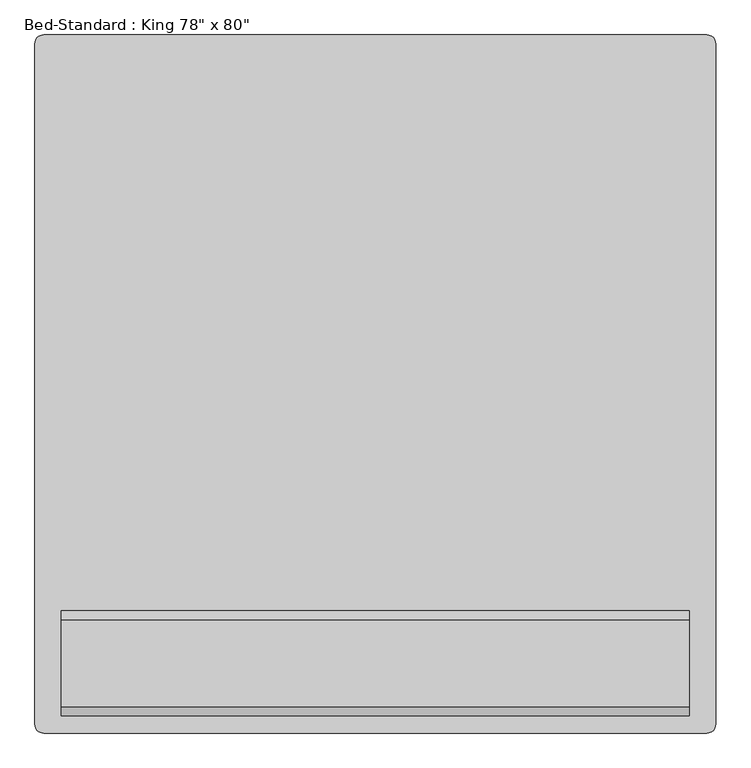
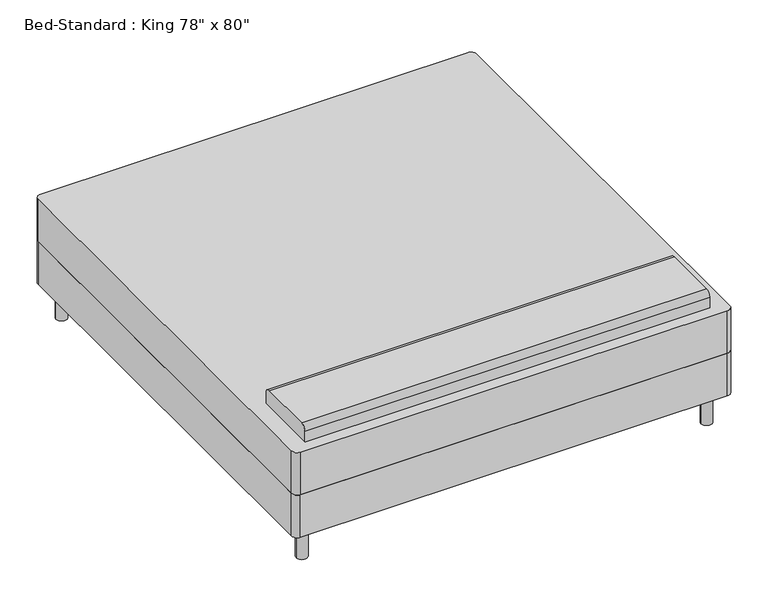
"""IFC4 building model written with IfcOpenShell, lengths in millimetres: furniture geometry."""

import ifcopenshell
import ifcopenshell.guid

model = None  # the IFC model being written
_history = None  # IfcOwnerHistory: only IFC2X3 demands one
_inside = {}  # id of a spatial element -> (the spatial element, [elements in it])
_under = {}  # id of a project, library or spatial element -> (it, [spatial elements below it])
_declared = {}  # id of a project -> (the project, [libraries it declares])
_typed = {}  # id of a type object -> (the type object, [elements of that type])
_made_of = {}  # id of a material, layer set ... -> (it, [elements and type objects made of it])


def new_model(schema):
    """Start an empty IFC model of exactly this schema.

    Asked for "IFC4X3", IfcOpenShell would pick the latest addendum, in which some entities
    have other attributes; the version numbers below select the first issue.
    IFC2X3 requires an IfcOwnerHistory on every rooted entity: one is made here for all.
    """
    global model, _history
    if schema == "IFC4X3":
        model = ifcopenshell.file(schema_version=(4, 3, 0, 0))
    else:
        model = ifcopenshell.file(schema=schema)
    _inside.clear()
    _under.clear()
    _declared.clear()
    _typed.clear()
    _made_of.clear()
    _history = None
    if model.schema == "IFC2X3":
        org = make("IfcOrganization", Name="unknown")
        user = make(
            "IfcPersonAndOrganization",
            ThePerson=make("IfcPerson", FamilyName="unknown"),
            TheOrganization=org,
        )
        app = make(
            "IfcApplication",
            ApplicationDeveloper=org,
            Version="unknown",
            ApplicationFullName="unknown",
            ApplicationIdentifier="unknown",
        )
        _history = make(
            "IfcOwnerHistory",
            OwningUser=user,
            OwningApplication=app,
            ChangeAction="ADDED",
            CreationDate=0,
        )
    return model


def make(cls, **values):
    """One entity of the class cls with the attributes given. An attribute that is None is left unset."""
    return model.create_entity(
        cls, **{name: value for name, value in values.items() if value is not None}
    )


def rooted(cls, **values):
    """An entity with a GlobalId (a new one), such as an element, a storey or a relation."""
    return make(cls, GlobalId=ifcopenshell.guid.new(), OwnerHistory=_history, **values)


def si_unit(unit_type, name, prefix=None):
    """IfcSIUnit, for example si_unit("LENGTHUNIT", "METRE", prefix="MILLI")."""
    return make("IfcSIUnit", UnitType=unit_type, Prefix=prefix, Name=name)


def assignment(units):
    """IfcUnitAssignment: the units of a project."""
    return None if units is None else make("IfcUnitAssignment", Units=units)


def point(xyz):
    """IfcCartesianPoint."""
    return None if xyz is None else make("IfcCartesianPoint", Coordinates=xyz)


def direction(xyz):
    """IfcDirection."""
    return None if xyz is None else make("IfcDirection", DirectionRatios=xyz)


def frame(location, z_axis=None, x_axis=None):
    """IfcAxis2Placement3D, a coordinate frame: its origin and axes. An axis left out is left unset."""
    return make(
        "IfcAxis2Placement3D",
        Location=point(location),
        Axis=direction(z_axis),
        RefDirection=direction(x_axis),
    )


def frame_2d(location, x_axis=None):
    """IfcAxis2Placement2D, a coordinate frame in the plane: its origin and x axis."""
    return make(
        "IfcAxis2Placement2D", Location=point(location), RefDirection=direction(x_axis)
    )


def origin():
    """The frame at (0, 0, 0) with its axes left unset."""
    return frame((0.0, 0.0, 0.0))


def origin_with_axes():
    """The frame at (0, 0, 0) with the z axis (0, 0, 1) and the x axis (1, 0, 0) written out."""
    return frame((0.0, 0.0, 0.0), z_axis=(0.0, 0.0, 1.0), x_axis=(1.0, 0.0, 0.0))


def place(relative_to, where):
    """IfcLocalPlacement: puts the frame where relative to a parent placement (None: the world)."""
    return make(
        "IfcLocalPlacement", PlacementRelTo=relative_to, RelativePlacement=where
    )


def context(
    kind, dimensions, precision=None, world=None, true_north=None, identifier=None
):
    """IfcGeometricRepresentationContext, for example the 3D "Model" context."""
    return make(
        "IfcGeometricRepresentationContext",
        ContextIdentifier=identifier,
        ContextType=kind,
        CoordinateSpaceDimension=dimensions,
        Precision=precision,
        WorldCoordinateSystem=world,
        TrueNorth=true_north,
    )


def project(units=None, contexts=None):
    """IfcProject with its units and contexts."""
    return rooted(
        "IfcProject",
        Name="project",
        RepresentationContexts=contexts,
        UnitsInContext=assignment(units),
    )


def spatial(cls, under=None, at=None, **own):
    """A site, building, storey or space (cls), placed at a placement, below another one or the project."""
    s = rooted(cls, ObjectPlacement=at, **own)
    if under is not None:
        _under.setdefault(under.id(), (under, []))[1].append(s)
    return s


def polyline(points):
    """IfcPolyline through the points."""
    return make("IfcPolyline", Points=[point(p) for p in points])


def circle_curve(where, radius):
    """IfcCircle in the frame where."""
    return make("IfcCircle", Position=where, Radius=radius)


def trimmed(basis, trim1, trim2, sense, master):
    """IfcTrimmedCurve: the piece of a basis curve between two trims."""
    return make(
        "IfcTrimmedCurve",
        BasisCurve=basis,
        Trim1=trim1,
        Trim2=trim2,
        SenseAgreement=sense,
        MasterRepresentation=master,
    )


def segment(curve, same_sense, transition):
    """IfcCompositeCurveSegment."""
    return make(
        "IfcCompositeCurveSegment",
        Transition=transition,
        SameSense=same_sense,
        ParentCurve=curve,
    )


def composite_curve(segments, self_intersect=None):
    """IfcCompositeCurve: segments joined end to end."""
    return make("IfcCompositeCurve", Segments=segments, SelfIntersect=self_intersect)


def outline(outer, holes=None, kind="AREA"):
    """IfcArbitraryClosedProfileDef: a profile drawn as a closed curve; with holes, ...WithVoids."""
    if holes is None:
        return make("IfcArbitraryClosedProfileDef", ProfileType=kind, OuterCurve=outer)
    return make(
        "IfcArbitraryProfileDefWithVoids",
        ProfileType=kind,
        OuterCurve=outer,
        InnerCurves=holes,
    )


def extrude(swept, where, along, depth):
    """IfcExtrudedAreaSolid: the profile swept, set in the frame where, extruded along a direction by depth."""
    return make(
        "IfcExtrudedAreaSolid",
        SweptArea=swept,
        Position=where,
        ExtrudedDirection=direction(along),
        Depth=depth,
    )


def shape(context_of_items, identifier, shape_type, items):
    """IfcShapeRepresentation: the items that make up one representation, for example the "Body"."""
    return make(
        "IfcShapeRepresentation",
        ContextOfItems=context_of_items,
        RepresentationIdentifier=identifier,
        RepresentationType=shape_type,
        Items=items,
    )


def source(mapping_origin, context_of_items, identifier, shape_type, items):
    """IfcRepresentationMap: a shape defined once, which mapped items show again and again."""
    return make(
        "IfcRepresentationMap",
        MappingOrigin=mapping_origin,
        MappedRepresentation=shape(context_of_items, identifier, shape_type, items),
    )


def transform(
    local_origin,
    x_axis=None,
    y_axis=None,
    z_axis=None,
    scale=None,
    scale2=None,
    scale3=None,
    uniform=True,
):
    """IfcCartesianTransformationOperator3D, or its non-uniform kind. x_axis, y_axis, z_axis: its Axis1, 2, 3."""
    if uniform:
        return make(
            "IfcCartesianTransformationOperator3D",
            Axis1=direction(x_axis),
            Axis2=direction(y_axis),
            LocalOrigin=point(local_origin),
            Scale=scale,
            Axis3=direction(z_axis),
        )
    return make(
        "IfcCartesianTransformationOperator3DnonUniform",
        Axis1=direction(x_axis),
        Axis2=direction(y_axis),
        LocalOrigin=point(local_origin),
        Scale=scale,
        Axis3=direction(z_axis),
        Scale2=scale2,
        Scale3=scale3,
    )


def mapped(mapping_source, mapping_target):
    """IfcMappedItem: shows the shape of a source again, moved by a transform."""
    return make(
        "IfcMappedItem", MappingSource=mapping_source, MappingTarget=mapping_target
    )


def made_of(thing, what):
    """Note that an element or type object is made of a material, layer set ...; save() writes the relation."""
    if what is not None:
        _made_of.setdefault(what.id(), (what, []))[1].append(thing)
    return thing


def element(
    cls,
    number,
    at=None,
    inside=None,
    cuts=None,
    type_object=None,
    material=None,
    context=None,
    identifier="Body",
    shape_type=None,
    held_by="IfcProductDefinitionShape",
    body=None,
    shapes=None,
    **own,
):
    """One element of the class cls, such as IfcWall. Its Tag is "e" and its number.

    at: its placement. inside: the storey or other place that contains it. cuts: it is an
    opening in that element (IfcRelVoidsElement). A single representation is given by context,
    identifier, shape_type and body (its items); several are given by shapes. held_by: the class
    of the entity that holds the representations. save() writes the other relations.
    """
    e = rooted(cls, Tag="e%d" % number, ObjectPlacement=at, **own)
    if body is not None:
        shapes = [shape(context, identifier, shape_type, body)]
    if shapes is not None:
        e.Representation = make(held_by, Representations=shapes)
    if inside is not None:
        _inside.setdefault(inside.id(), (inside, []))[1].append(e)
    if cuts is not None:
        rooted(
            "IfcRelVoidsElement", RelatingBuildingElement=cuts, RelatedOpeningElement=e
        )
    if type_object is not None:
        _typed.setdefault(type_object.id(), (type_object, []))[1].append(e)
    return made_of(e, material)


def aggregate(whole, parts):
    """IfcRelAggregates: a whole, such as a stair, and the parts it consists of."""
    return rooted("IfcRelAggregates", RelatingObject=whole, RelatedObjects=parts)


def save(model, path):
    """Write the relations noted so far, then the file.

    IfcRelAggregates (storeys below a building ...), IfcRelContainedInSpatialStructure (elements
    in a storey), IfcRelDefinesByType, IfcRelAssociatesMaterial and IfcRelDeclares: one each for
    every whole, place, type object, material and project.
    """
    for whole, parts in _under.values():
        aggregate(whole, parts)
    for where, things in _inside.values():
        rooted(
            "IfcRelContainedInSpatialStructure",
            RelatedElements=things,
            RelatingStructure=where,
        )
    for kind, things in _typed.values():
        rooted("IfcRelDefinesByType", RelatedObjects=things, RelatingType=kind)
    for what, things in _made_of.values():
        rooted("IfcRelAssociatesMaterial", RelatedObjects=things, RelatingMaterial=what)
    for by, libraries in _declared.values():
        rooted("IfcRelDeclares", RelatingContext=by, RelatedDefinitions=libraries)
    model.write(path)


def furniture_df776289(model_context):
    return source(origin(), model_context, "Body", "SweptSolid", [
        extrude(outline(composite_curve([segment(trimmed(circle_curve(frame_2d((-693.7114754, 1036.195082)), 25.4), [point((-719.1114754, 1036.195082))], [point((-693.7114754, 1061.595082))], False, "CARTESIAN"), True, "CONTINUOUS"), segment(polyline([(-693.7114754, 1061.595082), (1236.6885246, 1061.595082)]), True, "CONTINUOUS"), segment(trimmed(circle_curve(frame_2d((1236.6885246, 1036.195082)), 25.4), [point((1236.6885246, 1061.595082))], [point((1262.0885246, 1036.195082))], False, "CARTESIAN"), True, "CONTINUOUS"), segment(polyline([(1262.0885246, 1036.195082), (1262.0885246, -945.004918)]), True, "CONTINUOUS"), segment(trimmed(circle_curve(frame_2d((1236.6885246, -945.004918)), 25.4), [point((1262.0885246, -945.004918))], [point((1236.6885246, -970.404918))], False, "CARTESIAN"), True, "CONTINUOUS"), segment(polyline([(1236.6885246, -970.404918), (-693.7114754, -970.404918)]), True, "CONTINUOUS"), segment(trimmed(circle_curve(frame_2d((-693.7114754, -945.004918)), 25.4), [point((-693.7114754, -970.404918))], [point((-719.1114754, -945.004918))], False, "CARTESIAN"), True, "CONTINUOUS"), segment(polyline([(-719.1114754, -945.004918), (-719.1114754, 1036.195082)]), True, "CONTINUOUS")], self_intersect=False)), frame((0.0, 0.0, 152.4), z_axis=(0.0, 0.0, 1.0), x_axis=(1.0, 0.0, 0.0)), (0.0, 0.0, 1.0), 203.2),
        extrude(outline(composite_curve([segment(polyline([(-614.804918, 558.8), (-919.604918, 558.8), (-919.604918, 609.6)]), True, "CONTINUOUS"), segment(trimmed(circle_curve(frame_2d((-894.204918, 609.6)), 25.4), [point((-919.604918, 609.6))], [point((-894.204918, 635.0))], False, "CARTESIAN"), True, "CONTINUOUS"), segment(polyline([(-894.204918, 635.0), (-640.204918, 635.0)]), True, "CONTINUOUS"), segment(trimmed(circle_curve(frame_2d((-640.204918, 609.6)), 25.4), [point((-640.204918, 635.0))], [point((-614.804918, 609.6))], False, "CARTESIAN"), True, "CONTINUOUS"), segment(polyline([(-614.804918, 609.6), (-614.804918, 558.8)]), True, "CONTINUOUS")], self_intersect=False)), frame((-642.9114754, 0.0, 0.0), z_axis=(1.0, 0.0, 0.0), x_axis=(0.0, 1.0, 0.0)), (0.0, 0.0, 1.0), 1828.8),
        extrude(outline(composite_curve([segment(trimmed(circle_curve(frame_2d((-642.9114754, -894.204918)), 25.4), [point((-668.3114754, -894.204918))], [point((-617.5114754, -894.204918))], False, "CARTESIAN"), True, "CONTINUOUS"), segment(trimmed(circle_curve(frame_2d((-642.9114754, -894.204918)), 25.4), [point((-617.5114754, -894.204918))], [point((-668.3114754, -894.204918))], False, "CARTESIAN"), True, "CONTINUOUS")], self_intersect=False)), origin_with_axes(), (0.0, 0.0, 1.0), 152.4),
        extrude(outline(composite_curve([segment(trimmed(circle_curve(frame_2d((1185.8885246, -894.204918)), 25.4), [point((1160.4885246, -894.204918))], [point((1211.2885246, -894.204918))], False, "CARTESIAN"), True, "CONTINUOUS"), segment(trimmed(circle_curve(frame_2d((1185.8885246, -894.204918)), 25.4), [point((1211.2885246, -894.204918))], [point((1160.4885246, -894.204918))], False, "CARTESIAN"), True, "CONTINUOUS")], self_intersect=False)), origin_with_axes(), (0.0, 0.0, 1.0), 152.4),
        extrude(outline(composite_curve([segment(trimmed(circle_curve(frame_2d((1185.8885246, 985.395082)), 25.4), [point((1160.4885246, 985.395082))], [point((1211.2885246, 985.395082))], False, "CARTESIAN"), True, "CONTINUOUS"), segment(trimmed(circle_curve(frame_2d((1185.8885246, 985.395082)), 25.4), [point((1211.2885246, 985.395082))], [point((1160.4885246, 985.395082))], False, "CARTESIAN"), True, "CONTINUOUS")], self_intersect=False)), origin_with_axes(), (0.0, 0.0, 1.0), 152.4),
        extrude(outline(composite_curve([segment(trimmed(circle_curve(frame_2d((-642.9114754, 985.395082)), 25.4), [point((-668.3114754, 985.395082))], [point((-617.5114754, 985.395082))], False, "CARTESIAN"), True, "CONTINUOUS"), segment(trimmed(circle_curve(frame_2d((-642.9114754, 985.395082)), 25.4), [point((-617.5114754, 985.395082))], [point((-668.3114754, 985.395082))], False, "CARTESIAN"), True, "CONTINUOUS")], self_intersect=False)), origin_with_axes(), (0.0, 0.0, 1.0), 152.4),
        extrude(outline(composite_curve([segment(trimmed(circle_curve(frame_2d((-693.7114754, -945.004918)), 25.4), [point((-693.7114754, -970.404918))], [point((-719.1114754, -945.004918))], False, "CARTESIAN"), True, "CONTINUOUS"), segment(polyline([(-719.1114754, -945.004918), (-719.1114754, 1036.195082)]), True, "CONTINUOUS"), segment(trimmed(circle_curve(frame_2d((-693.7114754, 1036.195082)), 25.4), [point((-719.1114754, 1036.195082))], [point((-693.7114754, 1061.595082))], False, "CARTESIAN"), True, "CONTINUOUS"), segment(polyline([(-693.7114754, 1061.595082), (1236.6885246, 1061.595082)]), True, "CONTINUOUS"), segment(trimmed(circle_curve(frame_2d((1236.6885246, 1036.195082)), 25.4), [point((1236.6885246, 1061.595082))], [point((1262.0885246, 1036.195082))], False, "CARTESIAN"), True, "CONTINUOUS"), segment(polyline([(1262.0885246, 1036.195082), (1262.0885246, -945.004918)]), True, "CONTINUOUS"), segment(trimmed(circle_curve(frame_2d((1236.6885246, -945.004918)), 25.4), [point((1262.0885246, -945.004918))], [point((1236.6885246, -970.404918))], False, "CARTESIAN"), True, "CONTINUOUS"), segment(polyline([(1236.6885246, -970.404918), (-693.7114754, -970.404918)]), True, "CONTINUOUS")], self_intersect=False)), frame((0.0, 0.0, 355.6), z_axis=(0.0, 0.0, 1.0), x_axis=(1.0, 0.0, 0.0)), (0.0, 0.0, 1.0), 203.2),
    ])


if __name__ == "__main__":
    model = new_model("IFC4")
    model_context = context("Model", 3, world=origin())
    ifc_project = project(units=[si_unit("LENGTHUNIT", "METRE", prefix="MILLI")], contexts=[model_context])
    site = spatial("IfcSite", under=ifc_project)
    building = spatial("IfcBuilding", under=site)
    placement = place(None, origin())
    furniture_shape = furniture_df776289(model_context)
    element("IfcFurniture", 1, ObjectType="Bed-Standard : King 78\" x 80\"", at=placement, inside=building, context=model_context, shape_type="MappedRepresentation", body=[
        mapped(furniture_shape, transform((0.0, 0.0, 0.0), x_axis=(1.0, 0.0, 0.0), y_axis=(0.0, 1.0, 0.0), z_axis=(0.0, 0.0, 1.0))),
    ])
    save(model, "model.ifc")

# Revit data of these elements
# Type "Bed-Standard : King 78\" x 80\""
#   Assembly Code = "E2020200"
#   Clear Dim_2 = 2' - 0"
#   Clear Dim_1 = 3' - 0"
#   Length = 6' - 8"
#   Width = 6' - 6"
#   Leg Material = Metal - Chrome
#   Mattress Material = Textile - White
# Element 1 (IfcFurniture, "Bed-Standard : King 78\" x 80\"")
#   Materials on its faces: "Textile - White", "Metal - Chrome"
# Materials
#   "Metal - Chrome": class "Metal", colour RGB 17 17 17, transparency 0
#   "Textile - White": class "Fabric", colour RGB 247 247 239, transparency 0
